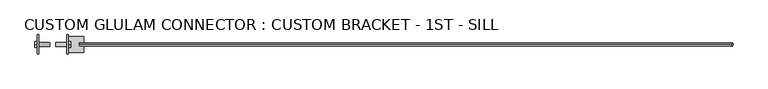
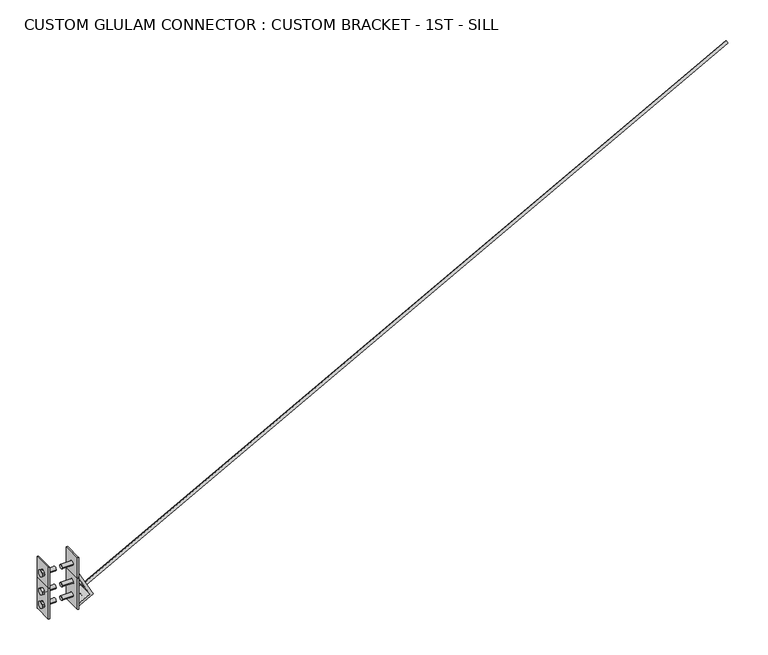
"""IFC4 building model written with IfcOpenShell, lengths in millimetres: fastener geometry, CUSTOM GLULAM CONNECTOR : CUSTOM BRACKET - 1ST - SILL."""

from ifc_helpers import new_model, si_unit, point, frame, frame_2d, origin, place, context, project, spatial, polyline, circle_curve, trimmed, segment, composite_curve, outline, extrude, source, transform, mapped, element, save
from ifc_brep_helpers import plane_surface, revolved_surface, advanced_brep


def custom_glulam_connector_custom_bracket_1st_sill_8d3b05b8(model_context):
    return source(origin(), model_context, "Body", "SolidModel", [
        advanced_brep(
        [(-87.3125, -13.890625, 160.3375), (-87.3125, 13.890625, 160.3375), (-95.25, 13.890625, 160.3375), (-95.25, -13.890625, 160.3375), (-95.25, 60.325, 211.1375), (-95.25, 60.325, 7.9375), (-95.25, 52.3875, 7.9375), (-95.25, -60.325, 7.9375), (-95.25, -60.325, 211.1375), (-95.25, 52.3875, 211.1375), (-95.25, 13.890625, 71.4375), (-95.25, -13.890625, 71.4375), (-87.3125, 13.890625, 71.4375), (-87.3125, -13.890625, 71.4375), (-87.3125, 60.325, 211.1375), (-87.3125, -60.325, 211.1375), (-87.3125, -60.325, 7.9375), (-87.3125, 60.325, 7.9375)],
        [
            (0, 1, circle_curve(frame((-87.3125, 0.0, 160.3375), z_axis=(1.0, 0.0, 0.0), x_axis=(0.0, 1.0, 0.0)), 13.890625)),
            (1, 2),
            (2, 3, circle_curve(frame((-95.25, 0.0, 160.3375), z_axis=(-1.0, 0.0, 0.0), x_axis=(0.0, 1.0, 0.0)), 13.890625)),
            (3, 0),
            (4, 5),
            (5, 6),
            (6, 7),
            (7, 8),
            (8, 9),
            (9, 4),
            (10, 11, circle_curve(frame((-95.25, 0.0, 71.4375), z_axis=(1.0, 0.0, 0.0), x_axis=(0.0, 1.0, 0.0)), 13.890625)),
            (11, 10, circle_curve(frame((-95.25, 0.0, 71.4375), z_axis=(1.0, 0.0, 0.0), x_axis=(0.0, 1.0, 0.0)), 13.890625)),
            (2, 3, circle_curve(frame((-95.25, 0.0, 160.3375), z_axis=(1.0, 0.0, 0.0), x_axis=(0.0, 1.0, 0.0)), 13.890625)),
            (10, 12),
            (12, 13, circle_curve(frame((-87.3125, 0.0, 71.4375), z_axis=(1.0, 0.0, 0.0), x_axis=(0.0, 1.0, 0.0)), 13.890625)),
            (13, 11),
            (1, 0, circle_curve(frame((-87.3125, 0.0, 160.3375), z_axis=(1.0, 0.0, 0.0), x_axis=(0.0, 1.0, 0.0)), 13.890625)),
            (13, 12, circle_curve(frame((-87.3125, 0.0, 71.4375), z_axis=(1.0, 0.0, 0.0), x_axis=(0.0, 1.0, 0.0)), 13.890625)),
            (14, 15),
            (15, 16),
            (16, 17),
            (17, 14),
            (8, 15),
            (14, 4),
            (7, 16),
            (5, 17),
        ],
        [
            revolved_surface(polyline([(-95.25, 13.890625, 160.3375), (-87.3125, 13.890625, 160.3375)]), (-87.3125, 0.0, 160.3375), (-1.0, 0.0, 0.0)),
            plane_surface(frame((-95.25, -60.325, 211.1375), z_axis=(-1.0, 0.0, 0.0), x_axis=(0.0, -1.0, 0.0))),
            revolved_surface(polyline([(-95.25, 13.890625, 71.4375), (-87.3125, 13.890625, 71.4375)]), (-87.3125, 0.0, 71.4375), (-1.0, 0.0, 0.0)),
            plane_surface(frame((-87.3125, -60.325, 211.1375), z_axis=(1.0, 0.0, 0.0), x_axis=(0.0, 1.0, 0.0))),
            plane_surface(frame((-95.25, 60.325, 211.1375), z_axis=(0.0, 0.0, 1.0), x_axis=(1.0, 0.0, 0.0))),
            plane_surface(frame((-95.25, -60.325, 211.1375), z_axis=(0.0, -1.0, 0.0), x_axis=(1.0, 0.0, 0.0))),
            plane_surface(frame((-95.25, -60.325, 7.9375), z_axis=(0.0, 0.0, -1.0), x_axis=(1.0, 0.0, 0.0))),
            plane_surface(frame((-95.25, 60.325, 7.9375), z_axis=(0.0, 1.0, 0.0), x_axis=(1.0, 0.0, 0.0))),
        ],
        [
            (0, [[1, 2, 3, 4]]),
            (1, [[5, 6, 7, 8, 9, 10], [11, 12], [13, -3]]),
            (2, [[-11, 14, 15, 16]]),
            (0, [[-13, -2, 17, -4]]),
            (2, [[18, -14, -12, -16]]),
            (3, [[19, 20, 21, 22], [-17, -1], [-15, -18]]),
            (4, [[23, -19, 24, -10, -9]]),
            (5, [[25, -20, -23, -8]]),
            (6, [[26, -21, -25, -7, -6]]),
            (7, [[-24, -22, -26, -5]]),
        ],
    ),
        extrude(outline(polyline([(-19.05, 171.3360226), (0.0, 182.3345453), (19.05, 171.3360226), (19.05, 149.3389774), (0.0, 138.3404547), (-19.05, 149.3389774), (-19.05, 171.3360226)])), frame((-110.2320312, 0.0, 0.0), z_axis=(1.0, 0.0, 0.0), x_axis=(0.0, 1.0, 0.0)), (0.0, 0.0, 1.0), 14.9820312),
        extrude(outline(composite_curve([segment(trimmed(circle_curve(frame_2d((0.0, 160.3375)), 12.7), [point((-12.7, 160.3375))], [point((12.7, 160.3375))], False, "CARTESIAN"), True, "CONTINUOUS"), segment(trimmed(circle_curve(frame_2d((0.0, 160.3375)), 12.7), [point((12.7, 160.3375))], [point((-12.7, 160.3375))], False, "CARTESIAN"), True, "CONTINUOUS")], self_intersect=False)), frame((-95.25, 0.0, 0.0), z_axis=(1.0, 0.0, 0.0), x_axis=(0.0, 1.0, 0.0)), (0.0, 0.0, 1.0), 76.2),
        extrude(outline(polyline([(-19.05, 82.4360226), (0.0, 93.4345453), (19.05, 82.4360226), (19.05, 60.4389774), (0.0, 49.4404547), (-19.05, 60.4389774), (-19.05, 82.4360226)])), frame((-110.2320312, 0.0, 0.0), z_axis=(1.0, 0.0, 0.0), x_axis=(0.0, 1.0, 0.0)), (0.0, 0.0, 1.0), 14.9820312),
        extrude(outline(composite_curve([segment(trimmed(circle_curve(frame_2d((0.0, 71.4375)), 12.7), [point((-12.7, 71.4375))], [point((12.7, 71.4375))], False, "CARTESIAN"), True, "CONTINUOUS"), segment(trimmed(circle_curve(frame_2d((0.0, 71.4375)), 12.7), [point((12.7, 71.4375))], [point((-12.7, 71.4375))], False, "CARTESIAN"), True, "CONTINUOUS")], self_intersect=False)), frame((-95.25, 0.0, 0.0), z_axis=(1.0, 0.0, 0.0), x_axis=(0.0, 1.0, 0.0)), (0.0, 0.0, 1.0), 76.2),
        extrude(outline(polyline([(-19.05, 171.3360226), (0.0, 182.3345453), (19.05, 171.3360226), (19.05, 149.3389774), (0.0, 138.3404547), (-19.05, 149.3389774), (-19.05, 171.3360226)])), frame((-110.2320312, 0.0, 0.0), z_axis=(1.0, 0.0, 0.0), x_axis=(0.0, 1.0, 0.0)), (0.0, 0.0, 1.0), 14.9820312),
        extrude(outline(composite_curve([segment(trimmed(circle_curve(frame_2d((0.0, 160.3375)), 12.7), [point((-12.7, 160.3375))], [point((12.7, 160.3375))], False, "CARTESIAN"), True, "CONTINUOUS"), segment(trimmed(circle_curve(frame_2d((0.0, 160.3375)), 12.7), [point((12.7, 160.3375))], [point((-12.7, 160.3375))], False, "CARTESIAN"), True, "CONTINUOUS")], self_intersect=False)), frame((-95.25, 0.0, 0.0), z_axis=(1.0, 0.0, 0.0), x_axis=(0.0, 1.0, 0.0)), (0.0, 0.0, 1.0), 76.2),
        advanced_brep(
        [(87.3125, -13.890625, 160.3375), (95.25, -13.890625, 160.3375), (95.25, 13.890625, 160.3375), (87.3125, 13.890625, 160.3375), (95.25, 60.325, 211.1375), (95.25, 52.3875, 211.1375), (95.25, -60.325, 211.1375), (95.25, -60.325, 7.9375), (95.25, 52.3875, 7.9375), (95.25, 60.325, 7.9375), (95.25, 13.890625, 71.4375), (95.25, -13.890625, 71.4375), (87.3125, -13.890625, 71.4375), (87.3125, 13.890625, 71.4375), (87.3125, 60.325, 211.1375), (87.3125, 60.325, 7.9375), (87.3125, -60.325, 7.9375), (87.3125, -60.325, 211.1375)],
        [
            (0, 1),
            (1, 2, circle_curve(frame((95.25, 0.0, 160.3375), z_axis=(1.0, 0.0, 0.0), x_axis=(0.0, 1.0, 0.0)), 13.890625)),
            (2, 3),
            (3, 0, circle_curve(frame((87.3125, 0.0, 160.3375), z_axis=(-1.0, 0.0, 0.0), x_axis=(0.0, 1.0, 0.0)), 13.890625)),
            (4, 5),
            (5, 6),
            (6, 7),
            (7, 8),
            (8, 9),
            (9, 4),
            (1, 2, circle_curve(frame((95.25, 0.0, 160.3375), z_axis=(-1.0, 0.0, 0.0), x_axis=(0.0, 1.0, 0.0)), 13.890625)),
            (10, 11, circle_curve(frame((95.25, 0.0, 71.4375), z_axis=(-1.0, 0.0, 0.0), x_axis=(0.0, 1.0, 0.0)), 13.890625)),
            (11, 10, circle_curve(frame((95.25, 0.0, 71.4375), z_axis=(-1.0, 0.0, 0.0), x_axis=(0.0, 1.0, 0.0)), 13.890625)),
            (11, 12),
            (12, 13, circle_curve(frame((87.3125, 0.0, 71.4375), z_axis=(-1.0, 0.0, 0.0), x_axis=(0.0, 1.0, 0.0)), 13.890625)),
            (13, 10),
            (0, 3, circle_curve(frame((87.3125, 0.0, 160.3375), z_axis=(-1.0, 0.0, 0.0), x_axis=(0.0, 1.0, 0.0)), 13.890625)),
            (13, 12, circle_curve(frame((87.3125, 0.0, 71.4375), z_axis=(-1.0, 0.0, 0.0), x_axis=(0.0, 1.0, 0.0)), 13.890625)),
            (14, 15),
            (15, 16),
            (16, 17),
            (17, 14),
            (4, 14),
            (17, 6),
            (16, 7),
            (15, 9),
        ],
        [
            revolved_surface(polyline([(95.25, 13.890625, 160.3375), (87.3125, 13.890625, 160.3375)]), (87.3125, 0.0, 160.3375), (1.0, 0.0, 0.0)),
            plane_surface(frame((95.25, -60.325, 211.1375), z_axis=(1.0, 0.0, 0.0), x_axis=(0.0, -1.0, 0.0))),
            revolved_surface(polyline([(95.25, 13.890625, 71.4375), (87.3125, 13.890625, 71.4375)]), (87.3125, 0.0, 71.4375), (1.0, 0.0, 0.0)),
            plane_surface(frame((87.3125, -60.325, 211.1375), z_axis=(-1.0, 0.0, 0.0), x_axis=(0.0, 1.0, 0.0))),
            plane_surface(frame((95.25, 60.325, 211.1375), z_axis=(0.0, 0.0, 1.0), x_axis=(-1.0, 0.0, 0.0))),
            plane_surface(frame((95.25, -60.325, 211.1375), z_axis=(0.0, -1.0, 0.0), x_axis=(-1.0, 0.0, 0.0))),
            plane_surface(frame((95.25, -60.325, 7.9375), z_axis=(0.0, 0.0, -1.0), x_axis=(-1.0, 0.0, 0.0))),
            plane_surface(frame((95.25, 60.325, 7.9375), z_axis=(0.0, 1.0, 0.0), x_axis=(-1.0, 0.0, 0.0))),
        ],
        [
            (0, [[1, 2, 3, 4]]),
            (1, [[5, 6, 7, 8, 9, 10], [-2, 11], [12, 13]]),
            (2, [[14, 15, 16, -13]]),
            (0, [[-1, 17, -3, -11]]),
            (2, [[-14, -12, -16, 18]]),
            (3, [[19, 20, 21, 22], [-4, -17], [-18, -15]]),
            (4, [[-6, -5, 23, -22, 24]]),
            (5, [[-7, -24, -21, 25]]),
            (6, [[-9, -8, -25, -20, 26]]),
            (7, [[-10, -26, -19, -23]]),
        ],
    ),
        extrude(outline(polyline([(-19.05, 171.3360226), (0.0, 182.3345453), (19.05, 171.3360226), (19.05, 149.3389774), (0.0, 138.3404547), (-19.05, 149.3389774), (-19.05, 171.3360226)])), frame((95.25, 0.0, 0.0), z_axis=(1.0, 0.0, 0.0), x_axis=(0.0, 1.0, 0.0)), (0.0, 0.0, 1.0), 14.9820312),
        extrude(outline(composite_curve([segment(trimmed(circle_curve(frame_2d((0.0, 160.3375)), 12.7), [point((-12.7, 160.3375))], [point((12.7, 160.3375))], False, "CARTESIAN"), True, "CONTINUOUS"), segment(trimmed(circle_curve(frame_2d((0.0, 160.3375)), 12.7), [point((12.7, 160.3375))], [point((-12.7, 160.3375))], False, "CARTESIAN"), True, "CONTINUOUS")], self_intersect=False)), frame((19.05, 0.0, 0.0), z_axis=(1.0, 0.0, 0.0), x_axis=(0.0, 1.0, 0.0)), (0.0, 0.0, 1.0), 76.2),
        extrude(outline(polyline([(-19.05, 82.4360226), (0.0, 93.4345453), (19.05, 82.4360226), (19.05, 60.4389774), (0.0, 49.4404547), (-19.05, 60.4389774), (-19.05, 82.4360226)])), frame((95.25, 0.0, 0.0), z_axis=(1.0, 0.0, 0.0), x_axis=(0.0, 1.0, 0.0)), (0.0, 0.0, 1.0), 14.9820312),
        extrude(outline(composite_curve([segment(trimmed(circle_curve(frame_2d((0.0, 71.4375)), 12.7), [point((-12.7, 71.4375))], [point((12.7, 71.4375))], False, "CARTESIAN"), True, "CONTINUOUS"), segment(trimmed(circle_curve(frame_2d((0.0, 71.4375)), 12.7), [point((12.7, 71.4375))], [point((-12.7, 71.4375))], False, "CARTESIAN"), True, "CONTINUOUS")], self_intersect=False)), frame((19.05, 0.0, 0.0), z_axis=(1.0, 0.0, 0.0), x_axis=(0.0, 1.0, 0.0)), (0.0, 0.0, 1.0), 76.2),
        extrude(outline(polyline([(-19.05, 171.3360226), (0.0, 182.3345453), (19.05, 171.3360226), (19.05, 149.3389774), (0.0, 138.3404547), (-19.05, 149.3389774), (-19.05, 171.3360226)])), frame((95.25, 0.0, 0.0), z_axis=(1.0, 0.0, 0.0), x_axis=(0.0, 1.0, 0.0)), (0.0, 0.0, 1.0), 14.9820312),
        extrude(outline(composite_curve([segment(trimmed(circle_curve(frame_2d((0.0, 160.3375)), 12.7), [point((-12.7, 160.3375))], [point((12.7, 160.3375))], False, "CARTESIAN"), True, "CONTINUOUS"), segment(trimmed(circle_curve(frame_2d((0.0, 160.3375)), 12.7), [point((12.7, 160.3375))], [point((-12.7, 160.3375))], False, "CARTESIAN"), True, "CONTINUOUS")], self_intersect=False)), frame((19.05, 0.0, 0.0), z_axis=(1.0, 0.0, 0.0), x_axis=(0.0, 1.0, 0.0)), (0.0, 0.0, 1.0), 76.2),
        advanced_brep(
        [(-95.25, 60.325, 350.8375), (-87.3125, 60.325, 350.8375), (-87.3125, 60.325, 211.1375), (-95.25, 60.325, 211.1375), (-87.3125, -13.890625, 280.9875), (-87.3125, 13.890625, 280.9875), (-95.25, 13.890625, 280.9875), (-95.25, -13.890625, 280.9875), (-95.25, -60.325, 350.8375), (-87.3125, -60.325, 350.8375), (-95.25, -52.3875, 350.8375), (-95.25, -52.3875, 211.1375), (-95.25, -60.325, 211.1375), (-87.3125, -60.325, 211.1375)],
        [
            (0, 1),
            (1, 2),
            (2, 3),
            (3, 0),
            (4, 5, circle_curve(frame((-87.3125, 0.0, 280.9875), z_axis=(1.0, 0.0, 0.0), x_axis=(0.0, 1.0, 0.0)), 13.890625)),
            (5, 6),
            (6, 7, circle_curve(frame((-95.25, 0.0, 280.9875), z_axis=(-1.0, 0.0, 0.0), x_axis=(0.0, 1.0, 0.0)), 13.890625)),
            (7, 4),
            (7, 6, circle_curve(frame((-95.25, 0.0, 280.9875), z_axis=(-1.0, 0.0, 0.0), x_axis=(0.0, 1.0, 0.0)), 13.890625)),
            (5, 4, circle_curve(frame((-87.3125, 0.0, 280.9875), z_axis=(1.0, 0.0, 0.0), x_axis=(0.0, 1.0, 0.0)), 13.890625)),
            (8, 9),
            (9, 1),
            (0, 10),
            (10, 8),
            (3, 11),
            (11, 12),
            (12, 8),
            (9, 13),
            (13, 2),
            (12, 13),
        ],
        [
            plane_surface(frame((-95.25, 60.325, 211.1375), z_axis=(0.0, 1.0, 0.0), x_axis=(1.0, 0.0, 0.0))),
            revolved_surface(polyline([(-95.25, 13.890625, 280.9875), (-87.3125, 13.890625, 280.9875)]), (-87.3125, 0.0, 280.9875), (-1.0, 0.0, 0.0)),
            plane_surface(frame((-95.25, 60.325, 350.8375), z_axis=(0.0, 0.0, 1.0), x_axis=(1.0, 0.0, 0.0))),
            plane_surface(frame((-95.25, -60.325, 350.8375), z_axis=(-1.0, 0.0, 0.0), x_axis=(0.0, -1.0, 0.0))),
            plane_surface(frame((-87.3125, -60.325, 350.8375), z_axis=(1.0, 0.0, 0.0), x_axis=(0.0, 1.0, 0.0))),
            plane_surface(frame((-95.25, -60.325, 350.8375), z_axis=(0.0, -1.0, 0.0), x_axis=(1.0, 0.0, 0.0))),
            plane_surface(frame((-95.25, -60.325, 211.1375), z_axis=(0.0, 0.0, -1.0), x_axis=(1.0, 0.0, 0.0))),
        ],
        [
            (0, [[1, 2, 3, 4]]),
            (1, [[5, 6, 7, 8]]),
            (1, [[9, -6, 10, -8]]),
            (2, [[11, 12, -1, 13, 14]]),
            (3, [[-4, 15, 16, 17, -14, -13], [-9, -7]]),
            (4, [[-12, 18, 19, -2], [-10, -5]]),
            (5, [[20, -18, -11, -17]]),
            (6, [[-3, -19, -20, -16, -15]]),
        ],
    ),
        extrude(outline(polyline([(-19.05, 291.9860226), (0.0, 302.9845453), (19.05, 291.9860226), (19.05, 269.9889774), (0.0, 258.9904547), (-19.05, 269.9889774), (-19.05, 291.9860226)])), frame((-110.2320312, 0.0, 0.0), z_axis=(1.0, 0.0, 0.0), x_axis=(0.0, 1.0, 0.0)), (0.0, 0.0, 1.0), 14.9820312),
        extrude(outline(composite_curve([segment(trimmed(circle_curve(frame_2d((0.0, 280.9875)), 12.7), [point((-12.7, 280.9875))], [point((12.7, 280.9875))], False, "CARTESIAN"), True, "CONTINUOUS"), segment(trimmed(circle_curve(frame_2d((0.0, 280.9875)), 12.7), [point((12.7, 280.9875))], [point((-12.7, 280.9875))], False, "CARTESIAN"), True, "CONTINUOUS")], self_intersect=False)), frame((-95.25, 0.0, 0.0), z_axis=(1.0, 0.0, 0.0), x_axis=(0.0, 1.0, 0.0)), (0.0, 0.0, 1.0), 76.2),
        advanced_brep(
        [(95.25, 60.325, 350.8375), (95.25, 60.325, 211.1375), (87.3125, 60.325, 211.1375), (87.3125, 60.325, 350.8375), (87.3125, -13.890625, 280.9875), (95.25, -13.890625, 280.9875), (95.25, 13.890625, 280.9875), (87.3125, 13.890625, 280.9875), (95.25, -60.325, 350.8375), (95.25, -52.3875, 350.8375), (87.3125, -60.325, 350.8375), (95.25, -60.325, 211.1375), (95.25, -52.3875, 211.1375), (87.3125, -60.325, 211.1375)],
        [
            (0, 1),
            (1, 2),
            (2, 3),
            (3, 0),
            (4, 5),
            (5, 6, circle_curve(frame((95.25, 0.0, 280.9875), z_axis=(1.0, 0.0, 0.0), x_axis=(0.0, 1.0, 0.0)), 13.890625)),
            (6, 7),
            (7, 4, circle_curve(frame((87.3125, 0.0, 280.9875), z_axis=(-1.0, 0.0, 0.0), x_axis=(0.0, 1.0, 0.0)), 13.890625)),
            (4, 7, circle_curve(frame((87.3125, 0.0, 280.9875), z_axis=(-1.0, 0.0, 0.0), x_axis=(0.0, 1.0, 0.0)), 13.890625)),
            (6, 5, circle_curve(frame((95.25, 0.0, 280.9875), z_axis=(1.0, 0.0, 0.0), x_axis=(0.0, 1.0, 0.0)), 13.890625)),
            (8, 9),
            (9, 0),
            (3, 10),
            (10, 8),
            (8, 11),
            (11, 12),
            (12, 1),
            (2, 13),
            (13, 10),
            (13, 11),
        ],
        [
            plane_surface(frame((95.25, 60.325, 211.1375), z_axis=(0.0, 1.0, 0.0), x_axis=(-1.0, 0.0, 0.0))),
            revolved_surface(polyline([(95.25, 13.890625, 280.9875), (87.3125, 13.890625, 280.9875)]), (87.3125, 0.0, 280.9875), (1.0, 0.0, 0.0)),
            plane_surface(frame((95.25, 60.325, 350.8375), z_axis=(0.0, 0.0, 1.0), x_axis=(-1.0, 0.0, 0.0))),
            plane_surface(frame((95.25, -60.325, 350.8375), z_axis=(1.0, 0.0, 0.0), x_axis=(0.0, -1.0, 0.0))),
            plane_surface(frame((87.3125, -60.325, 350.8375), z_axis=(-1.0, 0.0, 0.0), x_axis=(0.0, 1.0, 0.0))),
            plane_surface(frame((95.25, -60.325, 350.8375), z_axis=(0.0, -1.0, 0.0), x_axis=(-1.0, 0.0, 0.0))),
            plane_surface(frame((95.25, -60.325, 211.1375), z_axis=(0.0, 0.0, -1.0), x_axis=(-1.0, 0.0, 0.0))),
        ],
        [
            (0, [[1, 2, 3, 4]]),
            (1, [[5, 6, 7, 8]]),
            (1, [[-5, 9, -7, 10]]),
            (2, [[11, 12, -4, 13, 14]]),
            (3, [[-12, -11, 15, 16, 17, -1], [-6, -10]]),
            (4, [[-3, 18, 19, -13], [-8, -9]]),
            (5, [[-15, -14, -19, 20]]),
            (6, [[-17, -16, -20, -18, -2]]),
        ],
    ),
        extrude(outline(polyline([(-19.05, 291.9860226), (0.0, 302.9845453), (19.05, 291.9860226), (19.05, 269.9889774), (0.0, 258.9904547), (-19.05, 269.9889774), (-19.05, 291.9860226)])), frame((95.25, 0.0, 0.0), z_axis=(1.0, 0.0, 0.0), x_axis=(0.0, 1.0, 0.0)), (0.0, 0.0, 1.0), 14.9820312),
        extrude(outline(composite_curve([segment(trimmed(circle_curve(frame_2d((0.0, 280.9875)), 12.7), [point((-12.7, 280.9875))], [point((12.7, 280.9875))], False, "CARTESIAN"), True, "CONTINUOUS"), segment(trimmed(circle_curve(frame_2d((0.0, 280.9875)), 12.7), [point((12.7, 280.9875))], [point((-12.7, 280.9875))], False, "CARTESIAN"), True, "CONTINUOUS")], self_intersect=False)), frame((19.05, 0.0, 0.0), z_axis=(1.0, 0.0, 0.0), x_axis=(0.0, 1.0, 0.0)), (0.0, 0.0, 1.0), 76.2),
        extrude(outline(composite_curve([segment(trimmed(circle_curve(frame_2d((0.0, -9.525)), 9.525), [point((0.0, -19.05))], [point((0.0, 0.0))], False, "CARTESIAN"), True, "CONTINUOUS"), segment(trimmed(circle_curve(frame_2d((0.0, -9.525)), 9.525), [point((0.0, 0.0))], [point((0.0, -19.05))], False, "CARTESIAN"), True, "CONTINUOUS")], self_intersect=False)), frame((173.2138238, 0.0, 105.1724436), z_axis=(0.8788171126619665, 0.0, 0.4771587602596065), x_axis=(0.0, -1.0, 0.0)), (0.0, 0.0, 1.0), 4597.4),
        advanced_brep(
        [(192.9085516, -50.8, 68.8992672), (95.25, -50.8, 248.7639444), (95.25, -50.8, 215.4940952), (171.3824347, -50.8, 75.2755936), (95.25, -50.8, 33.9390543), (95.25, -50.8, 15.875), (192.9085516, 50.8, 68.8992672), (95.25, 50.8, 15.875), (95.25, 50.8, 33.9390543), (171.3824347, 50.8, 75.2755936), (95.25, 50.8, 215.4940952), (95.25, 50.8, 248.7639444), (173.781941, 0.0, 104.1261019), (163.5558323, 0.0, 122.9602512), (149.6046106, 0.0, 115.3853559), (159.8307193, 0.0, 96.5512066), (141.0385275, 0.0, 58.8001963), (140.3409665, 0.0, 58.4214515), (147.9158618, 0.0, 44.4702298), (148.6134229, 0.0, 44.8489746)],
        [
            (0, 1),
            (1, 2),
            (2, 3),
            (3, 4),
            (4, 5),
            (5, 0),
            (6, 7),
            (7, 8),
            (8, 9),
            (9, 10),
            (10, 11),
            (11, 6),
            (0, 6),
            (11, 1),
            (12, 13, circle_curve(frame((168.6688866, 0.0, 113.5431766), z_axis=(-0.8788171126619665, 0.0, -0.4771587602596065), x_axis=(-0.4771587602596065, 0.0, 0.8788171126619665)), 10.715625)),
            (13, 12, circle_curve(frame((168.6688866, 0.0, 113.5431766), z_axis=(-0.8788171126619665, 0.0, -0.4771587602596065), x_axis=(-0.4771587602596065, 0.0, 0.8788171126619665)), 10.715625)),
            (10, 2),
            (9, 3),
            (14, 15, circle_curve(frame((154.717665, 0.0, 105.9682812), z_axis=(0.8788171126619665, 0.0, 0.4771587602596065), x_axis=(-0.4771587602596065, 0.0, 0.8788171126619665)), 10.715625)),
            (15, 14, circle_curve(frame((154.717665, 0.0, 105.9682812), z_axis=(0.8788171126619665, 0.0, 0.4771587602596065), x_axis=(-0.4771587602596065, 0.0, 0.8788171126619665)), 10.715625)),
            (8, 4),
            (16, 17, circle_curve(frame((140.689747, 0.0, 58.6108239), z_axis=(0.47715876025960524, 0.0, -0.8788171126619673), x_axis=(0.878817112661967, 0.0, 0.47715876025960513)), 0.396875)),
            (17, 16, circle_curve(frame((140.689747, 0.0, 58.6108239), z_axis=(0.47715876025960524, 0.0, -0.8788171126619673), x_axis=(0.878817112661967, 0.0, 0.47715876025960513)), 0.396875)),
            (7, 5),
            (18, 19, circle_curve(frame((148.2646423, 0.0, 44.6596022), z_axis=(-0.47715876025960524, 0.0, 0.8788171126619673), x_axis=(0.878817112661967, 0.0, 0.47715876025960513)), 0.396875)),
            (19, 18, circle_curve(frame((148.2646423, 0.0, 44.6596022), z_axis=(-0.47715876025960524, 0.0, 0.8788171126619673), x_axis=(0.878817112661967, 0.0, 0.47715876025960513)), 0.396875)),
            (12, 15),
            (14, 13),
            (18, 17),
            (16, 19),
        ],
        [
            plane_surface(frame((95.25, -50.8, 248.7639444), z_axis=(0.0, -1.0000000000000002, 0.0), x_axis=(-0.4771587602596065, 0.0, 0.8788171126619665))),
            plane_surface(frame((95.25, 50.8, 248.7639444), z_axis=(0.0, 1.0000000000000002, 0.0), x_axis=(0.4771587602596065, 0.0, -0.8788171126619665))),
            plane_surface(frame((192.9085516, -50.8, 68.8992672), z_axis=(0.8788171126619665, 0.0, 0.4771587602596065), x_axis=(0.0, 1.0, 0.0))),
            plane_surface(frame((95.25, -50.8, 248.7639444), z_axis=(-1.0, 0.0, 0.0), x_axis=(0.0, 1.0, 0.0))),
            plane_surface(frame((95.25, -50.8, 215.4940952), z_axis=(-0.8788171126619664, 0.0, -0.4771587602596066), x_axis=(0.0, 1.0, 0.0))),
            plane_surface(frame((171.3824347, -50.8, 75.2755936), z_axis=(-0.4771587602596049, 0.0, 0.8788171126619674), x_axis=(0.0, 1.0, 0.0))),
            plane_surface(frame((95.25, -50.8, 33.9390543), z_axis=(-1.0, 0.0, 0.0), x_axis=(0.0, 1.0, 0.0))),
            plane_surface(frame((95.25, -50.8, 15.875), z_axis=(0.4771587602596052, 0.0, -0.8788171126619672), x_axis=(0.0, 1.0, 0.0))),
            revolved_surface(polyline([(149.60461058960067, 0.0, 115.38535590022673), (163.55583228121063, 0.0, 122.9602512346057)]), (168.6688866, 0.0, 113.5431766), (-0.8788171126619665, 0.0, -0.4771587602596065)),
            revolved_surface(polyline([(141.0385274949113, 0.0, 58.80019629723707), (148.61342285819435, 0.0, 44.848974552392434)]), (148.2646423, 0.0, 44.6596022), (-0.47715876025960513, 0.0, 0.878817112661967)),
        ],
        [
            (0, [[1, 2, 3, 4, 5, 6]]),
            (1, [[7, 8, 9, 10, 11, 12]]),
            (2, [[-1, 13, -12, 14], [15, 16]]),
            (3, [[-2, -14, -11, 17]]),
            (4, [[-3, -17, -10, 18], [19, 20]]),
            (5, [[-4, -18, -9, 21], [22, 23]]),
            (6, [[-5, -21, -8, 24]]),
            (7, [[-6, -24, -7, -13], [25, 26]]),
            (8, [[27, -19, 28, -15]]),
            (8, [[-27, -16, -28, -20]]),
            (9, [[29, -22, 30, -25]]),
            (9, [[-29, -26, -30, -23]]),
        ],
    ),
    ])


if __name__ == "__main__":
    model = new_model("IFC4")
    model_context = context("Model", 3, world=origin())
    ifc_project = project(units=[si_unit("LENGTHUNIT", "METRE", prefix="MILLI")], contexts=[model_context])
    site = spatial("IfcSite", under=ifc_project)
    building = spatial("IfcBuilding", under=site)
    placement = place(None, origin())
    custom_glulam_connector_custom_bracket_1st_sill_shape = custom_glulam_connector_custom_bracket_1st_sill_8d3b05b8(model_context)
    element("IfcFastener", 1, ObjectType="CUSTOM GLULAM CONNECTOR : CUSTOM BRACKET - 1ST - SILL", at=placement, inside=building, context=model_context, shape_type="MappedRepresentation", body=[
        mapped(custom_glulam_connector_custom_bracket_1st_sill_shape, transform((0.0, 0.0, 0.0), x_axis=(1.0, 0.0, 0.0), y_axis=(0.0, 1.0, 0.0), z_axis=(0.0, 0.0, 1.0))),
    ])
    save(model, "model.ifc")

# Revit data of these elements
# Type "CUSTOM GLULAM CONNECTOR : CUSTOM BRACKET - 1ST - SILL"
#   Width - Top = 0' - 6 7/8"
#   Top/Bottom Plate Thickness = 0' - 0 5/16"
#   Top/Bottom Plate - Width = 0' - 7 1/2"
#   Rod Radius = 0' - 0 3/8"
#   Rod Length [instance default] = 1' - 0"
#   Plate Thickness = 0' - 0 5/16"
#   Offset - Upper Plate 2 = 0' - 0"
#   Height of Plate = 0' - 8"
#   Width - Bottom = 0' - 6 7/8"
#   Plate Width = 0' - 4 3/4"
#   Bracket Width = 0' - 4"
#   Bracket Thickness = 0' - 0 5/8"
#   Bracket Offset in X = 0' - 3 3/4"
#   Bracket Offset in Y = 0' - 0 3/8"
#   Bracket Offset = 0' - 0 5/8"
#   Bracket Leg = 0' - 4 3/8"
#   Bracket Hole Radius - Up = 0' - 0 27/64"
#   Bracket Hole Radius - Down = 0' - 0 1/64"
#   Bracket Hole Offset = 0' - 2"
#   Beam Width = 0' - 7 3/8"
#   Angle 2 = 28.50°
#   Angle 1 = 118.50°
#   Top Plate Visible = no
#   Rod Visibility = yes
#   Plate Visibility - Upper Right 2 = no
#   Plate Visibility - Upper Right 1 = yes
#   Plate Visibility - Upper Left 2 = no
#   Plate Visibility - Upper Left 1 = yes
#   Plate Visibility - Lower Right 2 = no
#   Plate Visibility - Lower Right 1 = yes
#   Plate Visibility - Lower Left 2 = no
#   Plate Visibility - Lower Left 1 = yes
#   Bracket Visibility = yes
#   Bottom Plate Visible = no
#   Upper Plates - 2 = element 1323965
#   Upper Plates - 1 = element 1323965
#   Lower Plates = element 1339837
#   Bracket Material = 5/8" STEEL ANGLE (HDG AFTER FABRICATION)
#   URL = ""
# Element 1 (IfcFastener, "CUSTOM GLULAM CONNECTOR : CUSTOM BRACKET - 1ST - SILL")
#   Rod Length = 15' - 1"
#   Materials on its faces: "1\" GALV. LAG BOLT (LENGTH = 1/2\" SHY OF GLULAM DEPTH) -  (GALV. THRU BOLT IF PLATE ON OPP. SIDE OF STRUCT MEMBER)", "5/16\" STEEL PLATE (HDG AFTER FABRICATION)", "5/8\" STEEL ANGLE (HDG AFTER FABRICATION)", "3/4\" GALV. ROD (THREADED AT ENDS) - TURN BUCKLE AT 1/4 POINT OF TOTAL LENGTH"
# Materials
#   "5/8\" STEEL ANGLE (HDG AFTER FABRICATION)": class "Generic", colour RGB 195 195 195, transparency 0, Cost = 0
#   "1\" GALV. LAG BOLT (LENGTH = 1/2\" SHY OF GLULAM DEPTH) -  (GALV. THRU BOLT IF PLATE ON OPP. SIDE OF STRUCT MEMBER)": class "Generic", colour RGB 120 120 120, transparency 0, Cost = 0
#   "5/16\" STEEL PLATE (HDG AFTER FABRICATION)": class "Generic", colour RGB 232 232 232, transparency 0, Cost = 0
#   "3/4\" GALV. ROD (THREADED AT ENDS) - TURN BUCKLE AT 1/4 POINT OF TOTAL LENGTH": class "Generic", colour RGB 120 120 120, transparency 0, Cost = 0
